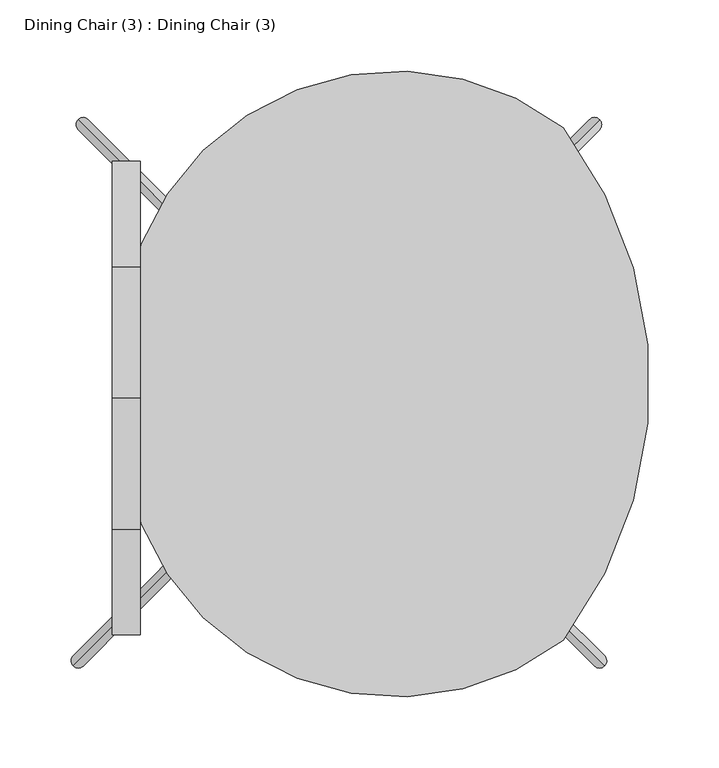
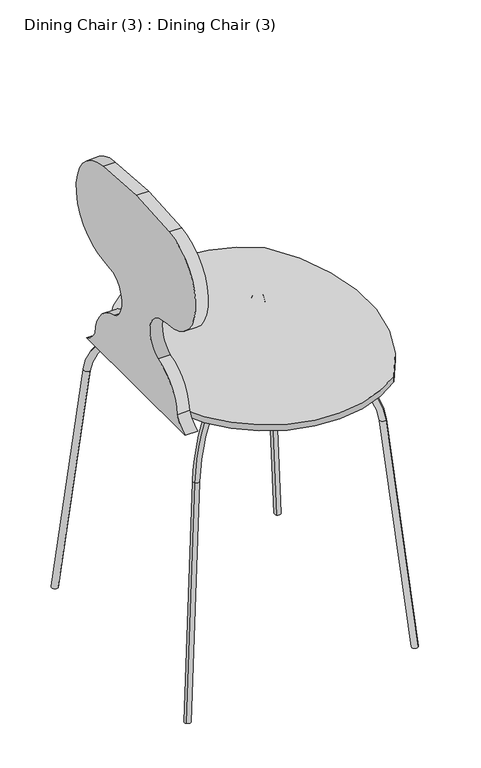
"""IFC4 building model written with IfcOpenShell, lengths in millimetres: furniture geometry, Dining Chair (3) : Dining Chair (3)."""

from ifc_helpers import new_model, si_unit, point, frame, frame_2d, origin, place, context, project, spatial, polyline, circle_curve, ellipse_curve, trimmed, segment, composite_curve, outline, extrude, source, transform, mapped, element, save
from ifc_brep_helpers import plane_surface, cylinder_surface, revolved_surface, advanced_brep


def dining_chair_3_dining_chair_3_7a8d451b(model_context):
    return source(origin(), model_context, "Body", "SolidModel", [
        extrude(outline(composite_curve([segment(trimmed(circle_curve(frame_2d((-359.6166368, 497.5978432)), 53.0867603), [point((-336.1081395, 450.0))], [point((-313.2599699, 471.7277146))], True, "CARTESIAN"), True, "CONTINUOUS"), segment(trimmed(circle_curve(frame_2d((-246.1723008, 468.3006658)), 67.1751442), [point((-313.2599699, 471.7277146))], [point((-259.8851361, 534.0612782))], False, "CARTESIAN"), True, "CONTINUOUS"), segment(trimmed(circle_curve(frame_2d((-276.1651573, 568.9730981)), 38.5210885), [point((-259.8851361, 534.0612782))], [point((-270.7823396, 607.1162434))], True, "CARTESIAN"), True, "CONTINUOUS"), segment(polyline([(-270.7823396, 607.1162434), (-287.8339558, 609.522593)]), True, "CONTINUOUS"), segment(trimmed(circle_curve(frame_2d((-285.7683653, 689.3681514)), 79.8722722), [point((-287.8339558, 609.522593))], [point((-291.3399734, 769.0458588))], False, "CARTESIAN"), True, "CONTINUOUS"), segment(polyline([(-291.3399734, 769.0458588), (-198.9971566, 775.5030976), (-106.6543399, 769.0458588)]), True, "CONTINUOUS"), segment(trimmed(circle_curve(frame_2d((-112.2259479, 689.3681514)), 79.8722722), [point((-106.6543399, 769.0458588))], [point((-110.1603574, 609.522593))], False, "CARTESIAN"), True, "CONTINUOUS"), segment(polyline([(-110.1603574, 609.522593), (-127.2119736, 607.1162434)]), True, "CONTINUOUS"), segment(trimmed(circle_curve(frame_2d((-121.8291559, 568.9730981)), 38.5210885), [point((-127.2119736, 607.1162434))], [point((-138.1091772, 534.0612782))], True, "CARTESIAN"), True, "CONTINUOUS"), segment(trimmed(circle_curve(frame_2d((-151.8220124, 468.3006658)), 67.1751442), [point((-138.1091772, 534.0612782))], [point((-84.7343434, 471.7277146))], False, "CARTESIAN"), True, "CONTINUOUS"), segment(trimmed(circle_curve(frame_2d((-38.3776765, 497.5978432)), 53.0867603), [point((-84.7343434, 471.7277146))], [point((-61.8861738, 450.0))], True, "CARTESIAN"), True, "CONTINUOUS"), segment(polyline([(-61.8861738, 450.0), (-336.1081395, 450.0)]), True, "CONTINUOUS")], self_intersect=False)), frame((22.7280076, 0.0, 0.0), z_axis=(1.0, 0.0, 0.0), x_axis=(0.0, 1.0, 0.0)), (0.0, 0.0, 1.0), 20.0),
        extrude(outline(composite_curve([segment(trimmed(circle_curve(frame_2d((222.4274135, -216.5279136)), 192.6164562), [point((340.0, -369.0985075))], [point((32.7280076, -249.9230424))], False, "CARTESIAN"), True, "CONTINUOUS"), segment(polyline([(32.7280076, -249.9230424), (32.7280076, -128.2739725)]), True, "CONTINUOUS"), segment(trimmed(circle_curve(frame_2d((222.4274135, -161.6691013)), 192.6164562), [point((32.7280076, -128.2739725))], [point((340.0, -9.0985075))], False, "CARTESIAN"), True, "CONTINUOUS"), segment(trimmed(circle_curve(frame_2d((103.3333333, -189.0985075)), 297.3400597), [point((340.0, -9.0985075))], [point((340.0, -369.0985075))], False, "CARTESIAN"), True, "CONTINUOUS")], self_intersect=False)), frame((0.0, 0.0, 450.0), z_axis=(0.0, 0.0, 1.0), x_axis=(1.0, 0.0, 0.0)), (0.0, 0.0, 1.0), 10.0),
        advanced_brep(
        [(361.9429089, -380.2370408, -0.6093467), (368.9612701, -387.255402, 0.6093467), (329.1794614, -347.4735933, 376.7549693), (336.1978225, -354.4919544, 377.9736627), (276.5417528, -294.8358847, 452.6147685), (276.5417528, -294.8358847, 442.6147685), (178.6593717, -196.9535036, 442.6147685), (178.6593717, -196.9535036, 452.6147685)],
        [
            (0, 1, circle_curve(frame((365.4520895, -383.7462214, 0.0), z_axis=(0.08617463914053405, -0.08617463914053361, -0.9925461516413217), x_axis=(0.7018361144661919, -0.701836114466188, 0.12186934340515031)), 5.0)),
            (1, 0, circle_curve(frame((365.4520895, -383.7462214, 0.0), z_axis=(0.08617463914053405, -0.08617463914053361, -0.9925461516413217), x_axis=(0.7018361144661919, -0.701836114466188, 0.12186934340515031)), 5.0)),
            (0, 2),
            (2, 3, circle_curve(frame((332.688642, -350.9827739, 377.364316), z_axis=(0.08617463914053405, -0.08617463914053361, -0.9925461516413217), x_axis=(0.7018361144661919, -0.701836114466188, 0.12186934340515031)), 5.0)),
            (3, 1),
            (3, 2, circle_curve(frame((332.688642, -350.9827739, 377.364316), z_axis=(0.08617463914053405, -0.08617463914053361, -0.9925461516413217), x_axis=(0.7018361144661919, -0.701836114466188, 0.12186934340515031)), 5.0)),
            (4, 3, circle_curve(frame((276.5417528, -294.8358847, 367.6147685), z_axis=(0.7071067811865457, 0.7071067811865495, 0.0), x_axis=(0.701836114466192, -0.7018361144661882, 0.12186934340514957)), 85.0)),
            (2, 5, circle_curve(frame((276.5417528, -294.8358847, 367.6147685), z_axis=(-0.7071067811865457, -0.7071067811865495, 0.0), x_axis=(0.701836114466192, -0.7018361144661882, 0.12186934340514957)), 75.0)),
            (5, 4, circle_curve(frame((276.5417528, -294.8358847, 447.6147685), z_axis=(0.7071067811865496, -0.7071067811865457, 0.0), x_axis=(0.0, 0.0, 1.0000000000000004)), 5.0)),
            (4, 5, circle_curve(frame((276.5417528, -294.8358847, 447.6147685), z_axis=(0.7071067811865496, -0.7071067811865457, 0.0), x_axis=(0.0, 0.0, 1.0000000000000004)), 5.0)),
            (6, 7, circle_curve(frame((178.6593717, -196.9535036, 447.6147685), z_axis=(-0.7071067811865493, 0.7071067811865457, 0.0), x_axis=(0.0, 0.0, 1.0)), 5.0)),
            (7, 6, circle_curve(frame((178.6593717, -196.9535036, 447.6147685), z_axis=(-0.7071067811865493, 0.7071067811865457, 0.0), x_axis=(0.0, 0.0, 1.0)), 5.0)),
            (5, 6),
            (7, 4),
        ],
        [
            plane_surface(frame((365.4520895, -383.7462214, 0.0), z_axis=(0.08617463914053401, -0.08617463914053357, -0.9925461516413218), x_axis=(-0.7071067811865457, -0.7071067811865493, 0.0))),
            cylinder_surface(frame((365.4520895, -383.7462214, 0.0), z_axis=(0.08617463914053407, -0.08617463914053362, -0.9925461516413219), x_axis=(0.7018361144661919, -0.701836114466188, 0.12186934340515031)), 5.0),
            revolved_surface(trimmed(ellipse_curve(frame((332.688642, -350.9827739, 377.364316), z_axis=(0.08617463914053365, -0.08617463914053322, -0.9925461516413222), x_axis=(0.7018361144661921, -0.7018361144661881, 0.12186934340514971)), 5.0, 5.0), [point((329.1794614, -347.4735933, 376.7549693))], [point((336.1978225, -354.4919544, 377.9736627))], True, "CARTESIAN"), (276.5417528, -294.8358847, 367.6147685), (-0.7071067811865458, -0.7071067811865496, 0.0)),
            revolved_surface(trimmed(ellipse_curve(frame((332.688642, -350.9827739, 377.364316), z_axis=(0.08617463914053365, -0.08617463914053322, -0.9925461516413222), x_axis=(0.7018361144661921, -0.7018361144661881, 0.12186934340514971)), 5.0, 5.0), [point((336.1978225, -354.4919544, 377.9736627))], [point((329.1794614, -347.4735933, 376.7549693))], True, "CARTESIAN"), (276.5417528, -294.8358847, 367.6147685), (-0.7071067811865458, -0.7071067811865496, 0.0)),
            plane_surface(frame((178.6593717, -196.9535036, 447.6147685), z_axis=(-0.7071067811865493, 0.7071067811865457, 0.0), x_axis=(-0.7071067811865457, -0.7071067811865493, 0.0))),
            cylinder_surface(frame((276.5417528, -294.8358847, 447.6147685), z_axis=(0.7071067811865493, -0.7071067811865457, 0.0), x_axis=(0.0, 0.0, 1.0)), 5.0),
        ],
        [
            (0, [[1, 2]]),
            (1, [[-1, 3, 4, 5]]),
            (1, [[-2, -5, 6, -3]]),
            (2, [[7, -4, 8, 9]]),
            (3, [[-8, -6, -7, 10]]),
            (4, [[11, 12]]),
            (5, [[-9, 13, -12, 14]]),
            (5, [[-10, -14, -11, -13]]),
        ],
    ),
        advanced_brep(
        [(358.407375, -10.1344324, -0.6093467), (365.4257362, -3.1160713, 0.6093467), (325.6439275, -42.89788, 376.7549693), (332.6622886, -35.8795188, 377.9736627), (273.0062189, -95.5355885, 452.6147685), (273.0062189, -95.5355885, 442.6147685), (175.1238378, -193.4179697, 442.6147685), (175.1238378, -193.4179697, 452.6147685)],
        [
            (0, 1, circle_curve(frame((361.9165556, -6.6252519, 0.0), z_axis=(0.08617463914053376, 0.08617463914053393, -0.9925461516413218), x_axis=(0.7018361144661892, 0.7018361144661905, 0.12186934340515031)), 5.0)),
            (1, 0, circle_curve(frame((361.9165556, -6.6252519, 0.0), z_axis=(0.08617463914053376, 0.08617463914053393, -0.9925461516413218), x_axis=(0.7018361144661892, 0.7018361144661905, 0.12186934340515031)), 5.0)),
            (0, 2),
            (2, 3, circle_curve(frame((329.1531081, -39.3886994, 377.364316), z_axis=(0.08617463914053376, 0.08617463914053393, -0.9925461516413218), x_axis=(0.7018361144661892, 0.7018361144661905, 0.12186934340515031)), 5.0)),
            (3, 1),
            (3, 2, circle_curve(frame((329.1531081, -39.3886994, 377.364316), z_axis=(0.08617463914053376, 0.08617463914053393, -0.9925461516413218), x_axis=(0.7018361144661892, 0.7018361144661905, 0.12186934340515031)), 5.0)),
            (4, 3, circle_curve(frame((273.0062189, -95.5355885, 367.6147685), z_axis=(-0.7071067811865482, 0.7071067811865469, 0.0), x_axis=(0.7018361144661893, 0.7018361144661907, 0.12186934340514957)), 85.0)),
            (2, 5, circle_curve(frame((273.0062189, -95.5355885, 367.6147685), z_axis=(0.7071067811865482, -0.7071067811865469, 0.0), x_axis=(0.7018361144661893, 0.7018361144661907, 0.12186934340514957)), 75.0)),
            (5, 4, circle_curve(frame((273.0062189, -95.5355885, 447.6147685), z_axis=(0.7071067811865469, 0.7071067811865482, 0.0), x_axis=(0.0, 0.0, 1.0000000000000002)), 5.0)),
            (4, 5, circle_curve(frame((273.0062189, -95.5355885, 447.6147685), z_axis=(0.7071067811865468, 0.7071067811865482, 0.0), x_axis=(0.0, 0.0, 1.0000000000000002)), 5.0)),
            (6, 7, circle_curve(frame((175.1238378, -193.4179697, 447.6147685), z_axis=(-0.7071067811865469, -0.7071067811865482, 0.0), x_axis=(0.0, 0.0, 1.0)), 5.0)),
            (7, 6, circle_curve(frame((175.1238378, -193.4179697, 447.6147685), z_axis=(-0.7071067811865469, -0.7071067811865482, 0.0), x_axis=(0.0, 0.0, 1.0)), 5.0)),
            (5, 6),
            (7, 4),
        ],
        [
            plane_surface(frame((361.9165556, -6.6252519, 0.0), z_axis=(0.0861746391405337, 0.08617463914053386, -0.9925461516413218), x_axis=(0.7071067811865482, -0.7071067811865469, 0.0))),
            cylinder_surface(frame((361.9165556, -6.6252519, 0.0), z_axis=(0.08617463914053376, 0.08617463914053393, -0.9925461516413218), x_axis=(0.7018361144661892, 0.7018361144661905, 0.12186934340515031)), 5.0),
            revolved_surface(trimmed(ellipse_curve(frame((329.1531081, -39.3886994, 377.364316), z_axis=(0.08617463914053337, 0.08617463914053354, -0.9925461516413219), x_axis=(0.7018361144661893, 0.7018361144661907, 0.12186934340514977)), 5.0, 5.0), [point((325.6439275, -42.89788, 376.7549693))], [point((332.6622886, -35.8795188, 377.9736627))], True, "CARTESIAN"), (273.0062189, -95.5355885, 367.6147685), (0.7071067811865482, -0.7071067811865469, 0.0)),
            revolved_surface(trimmed(ellipse_curve(frame((329.1531081, -39.3886994, 377.364316), z_axis=(0.08617463914053337, 0.08617463914053354, -0.9925461516413219), x_axis=(0.7018361144661893, 0.7018361144661907, 0.12186934340514977)), 5.0, 5.0), [point((332.6622886, -35.8795188, 377.9736627))], [point((325.6439275, -42.89788, 376.7549693))], True, "CARTESIAN"), (273.0062189, -95.5355885, 367.6147685), (0.7071067811865482, -0.7071067811865469, 0.0)),
            plane_surface(frame((175.1238378, -193.4179697, 447.6147685), z_axis=(-0.7071067811865468, -0.7071067811865482, 0.0), x_axis=(0.7071067811865482, -0.7071067811865468, 0.0))),
            cylinder_surface(frame((273.0062189, -95.5355885, 447.6147685), z_axis=(0.7071067811865469, 0.7071067811865482, 0.0), x_axis=(0.0, 0.0, 1.0)), 5.0),
        ],
        [
            (0, [[1, 2]]),
            (1, [[-1, 3, 4, 5]]),
            (1, [[-2, -5, 6, -3]]),
            (2, [[7, -4, 8, 9]]),
            (3, [[-8, -6, -7, 10]]),
            (4, [[11, 12]]),
            (5, [[-9, 13, -12, 14]]),
            (5, [[-10, -14, -11, -13]]),
        ],
    ),
        advanced_brep(
        [(2.4469023, -380.2370408, -0.6093467), (-4.5714589, -387.255402, 0.6093467), (35.2103498, -347.4735933, 376.7549693), (28.1919886, -354.4919544, 377.9736627), (87.8480584, -294.8358847, 452.6147685), (87.8480584, -294.8358847, 442.6147685), (185.7304395, -196.9535036, 442.6147685), (185.7304395, -196.9535036, 452.6147685)],
        [
            (0, 1, circle_curve(frame((-1.0622783, -383.7462214, 0.0), z_axis=(-0.08617463914053405, -0.08617463914053361, -0.9925461516413217), x_axis=(-0.7018361144661919, -0.701836114466188, 0.12186934340515031)), 5.0)),
            (1, 0, circle_curve(frame((-1.0622783, -383.7462214, 0.0), z_axis=(-0.08617463914053405, -0.08617463914053361, -0.9925461516413217), x_axis=(-0.7018361144661919, -0.701836114466188, 0.12186934340515031)), 5.0)),
            (0, 2),
            (2, 3, circle_curve(frame((31.7011692, -350.9827739, 377.364316), z_axis=(-0.08617463914053405, -0.08617463914053361, -0.9925461516413217), x_axis=(-0.7018361144661919, -0.701836114466188, 0.12186934340515031)), 5.0)),
            (3, 1),
            (3, 2, circle_curve(frame((31.7011692, -350.9827739, 377.364316), z_axis=(-0.08617463914053405, -0.08617463914053361, -0.9925461516413217), x_axis=(-0.7018361144661919, -0.701836114466188, 0.12186934340515031)), 5.0)),
            (4, 3, circle_curve(frame((87.8480584, -294.8358847, 367.6147685), z_axis=(0.7071067811865457, -0.7071067811865495, 0.0), x_axis=(-0.701836114466192, -0.7018361144661882, 0.12186934340514957)), 85.0)),
            (2, 5, circle_curve(frame((87.8480584, -294.8358847, 367.6147685), z_axis=(-0.7071067811865457, 0.7071067811865495, 0.0), x_axis=(-0.701836114466192, -0.7018361144661882, 0.12186934340514957)), 75.0)),
            (5, 4, circle_curve(frame((87.8480584, -294.8358847, 447.6147685), z_axis=(-0.7071067811865496, -0.7071067811865458, 0.0), x_axis=(0.0, 0.0, 1.0000000000000004)), 5.0)),
            (4, 5, circle_curve(frame((87.8480584, -294.8358847, 447.6147685), z_axis=(-0.7071067811865496, -0.7071067811865457, 0.0), x_axis=(0.0, 0.0, 1.0000000000000004)), 5.0)),
            (6, 7, circle_curve(frame((185.7304395, -196.9535036, 447.6147685), z_axis=(0.7071067811865493, 0.7071067811865457, 0.0), x_axis=(0.0, 0.0, 1.0)), 5.0)),
            (7, 6, circle_curve(frame((185.7304395, -196.9535036, 447.6147685), z_axis=(0.7071067811865493, 0.7071067811865457, 0.0), x_axis=(0.0, 0.0, 1.0)), 5.0)),
            (5, 6),
            (7, 4),
        ],
        [
            plane_surface(frame((-1.0622783, -383.7462214, 0.0), z_axis=(-0.08617463914053401, -0.08617463914053357, -0.9925461516413218), x_axis=(0.7071067811865457, -0.7071067811865493, 0.0))),
            cylinder_surface(frame((-1.0622783, -383.7462214, 0.0), z_axis=(-0.08617463914053407, -0.08617463914053362, -0.9925461516413219), x_axis=(-0.7018361144661919, -0.701836114466188, 0.12186934340515031)), 5.0),
            revolved_surface(trimmed(ellipse_curve(frame((31.7011692, -350.9827739, 377.364316), z_axis=(-0.08617463914053365, -0.08617463914053322, -0.9925461516413222), x_axis=(-0.7018361144661921, -0.7018361144661881, 0.12186934340514971)), 5.0, 5.0), [point((35.2103498, -347.4735933, 376.7549693))], [point((28.1919886, -354.4919544, 377.9736627))], True, "CARTESIAN"), (87.8480584, -294.8358847, 367.6147685), (-0.7071067811865458, 0.7071067811865496, 0.0)),
            revolved_surface(trimmed(ellipse_curve(frame((31.7011692, -350.9827739, 377.364316), z_axis=(-0.08617463914053365, -0.08617463914053322, -0.9925461516413222), x_axis=(-0.7018361144661921, -0.7018361144661881, 0.12186934340514971)), 5.0, 5.0), [point((28.1919886, -354.4919544, 377.9736627))], [point((35.2103498, -347.4735933, 376.7549693))], True, "CARTESIAN"), (87.8480584, -294.8358847, 367.6147685), (-0.7071067811865458, 0.7071067811865496, 0.0)),
            plane_surface(frame((185.7304395, -196.9535036, 447.6147685), z_axis=(0.7071067811865493, 0.7071067811865457, 0.0), x_axis=(0.7071067811865457, -0.7071067811865493, 0.0))),
            cylinder_surface(frame((87.8480584, -294.8358847, 447.6147685), z_axis=(-0.7071067811865493, -0.7071067811865457, 0.0), x_axis=(0.0, 0.0, 1.0)), 5.0),
        ],
        [
            (0, [[1, 2]]),
            (1, [[-1, 3, 4, 5]]),
            (1, [[-2, -5, 6, -3]]),
            (2, [[7, -4, 8, 9]]),
            (3, [[-8, -6, -7, 10]]),
            (4, [[11, 12]]),
            (5, [[-9, 13, -12, 14]]),
            (5, [[-10, -14, -11, -13]]),
        ],
    ),
        advanced_brep(
        [(5.9824362, -10.1344324, -0.6093467), (-1.035925, -3.1160713, 0.6093467), (38.7458837, -42.89788, 376.7549693), (31.7275226, -35.8795188, 377.9736627), (91.3835923, -95.5355885, 452.6147685), (91.3835923, -95.5355885, 442.6147685), (189.2659734, -193.4179697, 442.6147685), (189.2659734, -193.4179697, 452.6147685)],
        [
            (0, 1, circle_curve(frame((2.4732556, -6.6252519, 0.0), z_axis=(-0.08617463914053376, 0.08617463914053393, -0.9925461516413218), x_axis=(-0.7018361144661892, 0.7018361144661905, 0.12186934340515031)), 5.0)),
            (1, 0, circle_curve(frame((2.4732556, -6.6252519, 0.0), z_axis=(-0.08617463914053376, 0.08617463914053393, -0.9925461516413218), x_axis=(-0.7018361144661892, 0.7018361144661905, 0.12186934340515031)), 5.0)),
            (0, 2),
            (2, 3, circle_curve(frame((35.2367031, -39.3886994, 377.364316), z_axis=(-0.08617463914053376, 0.08617463914053393, -0.9925461516413218), x_axis=(-0.7018361144661892, 0.7018361144661905, 0.12186934340515031)), 5.0)),
            (3, 1),
            (3, 2, circle_curve(frame((35.2367031, -39.3886994, 377.364316), z_axis=(-0.08617463914053376, 0.08617463914053393, -0.9925461516413218), x_axis=(-0.7018361144661892, 0.7018361144661905, 0.12186934340515031)), 5.0)),
            (4, 3, circle_curve(frame((91.3835923, -95.5355885, 367.6147685), z_axis=(-0.7071067811865482, -0.7071067811865469, 0.0), x_axis=(-0.7018361144661893, 0.7018361144661907, 0.12186934340514957)), 85.0)),
            (2, 5, circle_curve(frame((91.3835923, -95.5355885, 367.6147685), z_axis=(0.7071067811865482, 0.7071067811865469, 0.0), x_axis=(-0.7018361144661893, 0.7018361144661907, 0.12186934340514957)), 75.0)),
            (5, 4, circle_curve(frame((91.3835923, -95.5355885, 447.6147685), z_axis=(-0.7071067811865469, 0.7071067811865482, 0.0), x_axis=(0.0, 0.0, 1.0000000000000002)), 5.0)),
            (4, 5, circle_curve(frame((91.3835923, -95.5355885, 447.6147685), z_axis=(-0.7071067811865469, 0.7071067811865482, 0.0), x_axis=(0.0, 0.0, 1.0000000000000002)), 5.0)),
            (6, 7, circle_curve(frame((189.2659734, -193.4179697, 447.6147685), z_axis=(0.7071067811865469, -0.7071067811865482, 0.0), x_axis=(0.0, 0.0, 1.0)), 5.0)),
            (7, 6, circle_curve(frame((189.2659734, -193.4179697, 447.6147685), z_axis=(0.7071067811865469, -0.7071067811865482, 0.0), x_axis=(0.0, 0.0, 1.0)), 5.0)),
            (5, 6),
            (7, 4),
        ],
        [
            plane_surface(frame((2.4732556, -6.6252519, 0.0), z_axis=(-0.0861746391405337, 0.08617463914053386, -0.9925461516413218), x_axis=(-0.7071067811865482, -0.7071067811865469, 0.0))),
            cylinder_surface(frame((2.4732556, -6.6252519, 0.0), z_axis=(-0.08617463914053376, 0.08617463914053393, -0.9925461516413218), x_axis=(-0.7018361144661892, 0.7018361144661905, 0.12186934340515031)), 5.0),
            revolved_surface(trimmed(ellipse_curve(frame((35.2367031, -39.3886994, 377.364316), z_axis=(-0.08617463914053337, 0.08617463914053354, -0.9925461516413219), x_axis=(-0.7018361144661893, 0.7018361144661907, 0.12186934340514977)), 5.0, 5.0), [point((38.7458837, -42.89788, 376.7549693))], [point((31.7275226, -35.8795188, 377.9736627))], True, "CARTESIAN"), (91.3835923, -95.5355885, 367.6147685), (0.7071067811865482, 0.7071067811865469, 0.0)),
            revolved_surface(trimmed(ellipse_curve(frame((35.2367031, -39.3886994, 377.364316), z_axis=(-0.08617463914053337, 0.08617463914053354, -0.9925461516413219), x_axis=(-0.7018361144661893, 0.7018361144661907, 0.12186934340514977)), 5.0, 5.0), [point((31.7275226, -35.8795188, 377.9736627))], [point((38.7458837, -42.89788, 376.7549693))], True, "CARTESIAN"), (91.3835923, -95.5355885, 367.6147685), (0.7071067811865482, 0.7071067811865469, 0.0)),
            plane_surface(frame((189.2659734, -193.4179697, 447.6147685), z_axis=(0.7071067811865468, -0.7071067811865482, 0.0), x_axis=(-0.7071067811865482, -0.7071067811865468, 0.0))),
            cylinder_surface(frame((91.3835923, -95.5355885, 447.6147685), z_axis=(-0.7071067811865469, 0.7071067811865482, 0.0), x_axis=(0.0, 0.0, 1.0)), 5.0),
        ],
        [
            (0, [[1, 2]]),
            (1, [[-1, 3, 4, 5]]),
            (1, [[-2, -5, 6, -3]]),
            (2, [[7, -4, 8, 9]]),
            (3, [[-8, -6, -7, 10]]),
            (4, [[11, 12]]),
            (5, [[-9, 13, -12, 14]]),
            (5, [[-10, -14, -11, -13]]),
        ],
    ),
    ])


if __name__ == "__main__":
    model = new_model("IFC4")
    model_context = context("Model", 3, world=origin())
    ifc_project = project(units=[si_unit("LENGTHUNIT", "METRE", prefix="MILLI")], contexts=[model_context])
    site = spatial("IfcSite", under=ifc_project)
    building = spatial("IfcBuilding", under=site)
    placement = place(None, origin())
    dining_chair_3_dining_chair_3_shape = dining_chair_3_dining_chair_3_7a8d451b(model_context)
    element("IfcFurniture", 1, ObjectType="Dining Chair (3) : Dining Chair (3)", at=placement, inside=building, context=model_context, shape_type="MappedRepresentation", body=[
        mapped(dining_chair_3_dining_chair_3_shape, transform((0.0, 0.0, 0.0), x_axis=(1.0, 0.0, 0.0), y_axis=(0.0, 1.0, 0.0), z_axis=(0.0, 0.0, 1.0))),
    ])
    save(model, "model.ifc")

# Revit data of these elements
# Type "Dining Chair (3) : Dining Chair (3)"
#   Keynote = "12600"
#   Bracket Material = Herman Miller - Finish 47 Trivalent Chrome
#   Cushion/Chair Back Material = Herman Miller - Veneer Z5 Maple
#   Manufacturer = ""
#   Model = ""
# Element 1 (IfcFurniture, "Dining Chair (3) : Dining Chair (3)")
#   Materials on its faces: "Herman Miller - Finish 47 Trivalent Chrome", "Herman Miller - Veneer Z5 Maple"
# Materials
#   "Herman Miller - Finish 47 Trivalent Chrome": class "Plastic", colour RGB 244 244 244, transparency 0, Keynote = "﻿﻿               ​      ​   ​  ​  ﻿     ﻿   ﻿      ﻿     ​                      ​      ​       ﻿  ﻿   ﻿​  ​​   ​​ ​                                 ﻿                  ​​​   ​  ​   ﻿ ﻿        ﻿﻿                            ​ ​                           ​          ​       ﻿  ﻿          ﻿             ﻿                   ﻿﻿", Comments = "﻿﻿               ​      ​   ​  ​  ﻿     ﻿   ﻿      ﻿     ​                      ​      ​       ﻿  ﻿   ﻿​  ​​   ​​ ​                                 ﻿                  ​​​   ​  ​   ﻿ ﻿        ﻿﻿                            ​ ​                           ​          ​       ﻿  ﻿          ﻿             ﻿                   ﻿﻿", Description = "﻿﻿               ​      ​   ​  ​  ﻿     ﻿   ﻿      ﻿     ​                      ​      ​       ﻿  ﻿   ﻿​  ​​   ​​ ​                                 ﻿                  ​​​   ​  ​   ﻿ ﻿        ﻿﻿                            ​ ​                           ​          ​       ﻿  ﻿          ﻿             ﻿                   ﻿﻿", Cost = 0
#   "Herman Miller - Veneer Z5 Maple": class "Unassigned", colour RGB 116 94 80, transparency 0, Keynote = "﻿﻿         ​             ﻿ ﻿ ﻿                 ​             ﻿         ​       ​  ﻿​       ﻿ ﻿   ﻿                     ​        ​  ​      ​  ​            ​﻿                      ​       ​﻿            ​      ﻿﻿​​                ﻿             ​  ​               ​﻿  ﻿                                          ​ ​​​​ ​       ﻿﻿", Comments = "﻿﻿         ​             ﻿ ﻿ ﻿                 ​             ﻿         ​       ​  ﻿​       ﻿ ﻿   ﻿                     ​        ​  ​      ​  ​            ​﻿                      ​       ​﻿            ​      ﻿﻿​​                ﻿             ​  ​               ​﻿  ﻿                                          ​ ​​​​ ​       ﻿﻿", Description = "﻿﻿         ​             ﻿ ﻿ ﻿                 ​             ﻿         ​       ​  ﻿​       ﻿ ﻿   ﻿                     ​        ​  ​      ​  ​            ​﻿                      ​       ​﻿            ​      ﻿﻿​​                ﻿             ​  ​               ​﻿  ﻿                                          ​ ​​​​ ​       ﻿﻿", Cost = 0
